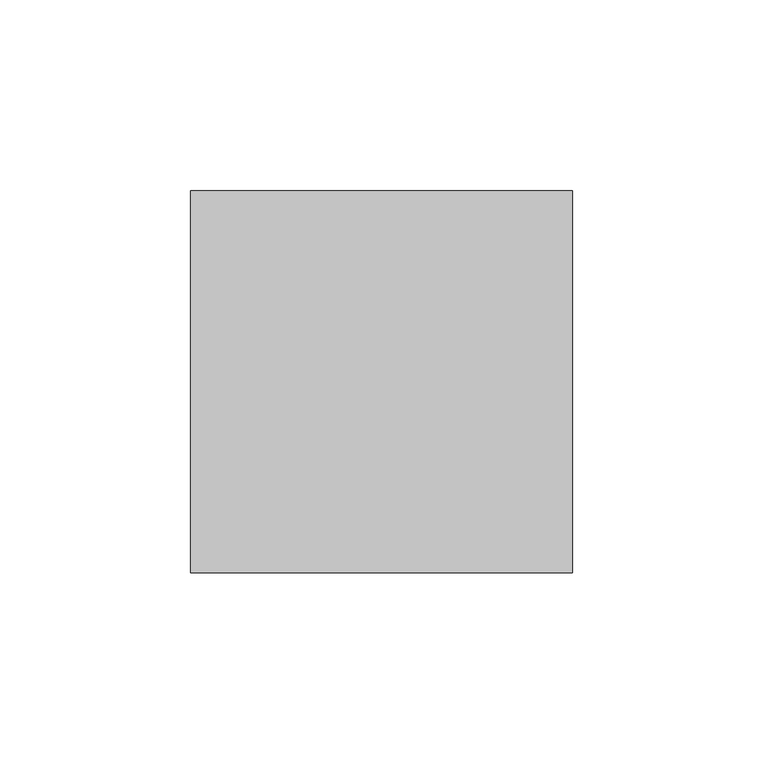
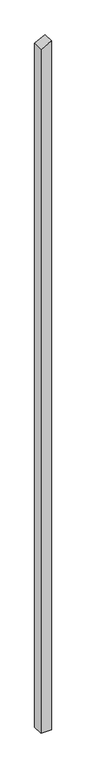
"""IFC4 building model written with IfcOpenShell, lengths in millimetres: column geometry, Holzstütze 160056 : Holzstütze 160056."""

from ifc_helpers import new_model, si_unit, frame, origin, place, context, project, spatial, polyline, outline, extrude, source, transform, mapped, element, save


def column_f815af80(model_context):
    return source(origin(), model_context, "Body", "SweptSolid", [
        extrude(outline(polyline([(-500.0, 157297.7593015), (-500.0, 157397.7593015), (6396.6643707, 157397.7593015), (6345.7118258, 157297.7593015), (-500.0, 157297.7593015)])), frame((0.0, 31941.5369795, 0.0), z_axis=(0.0, 1.0, 0.0), x_axis=(0.0, 0.0, 1.0)), (0.0, 0.0, 1.0), 100.0),
    ])


if __name__ == "__main__":
    model = new_model("IFC4")
    model_context = context("Model", 3, world=origin())
    ifc_project = project(units=[si_unit("LENGTHUNIT", "METRE", prefix="MILLI")], contexts=[model_context])
    site = spatial("IfcSite", under=ifc_project)
    building = spatial("IfcBuilding", under=site)
    placement = place(None, origin())
    column_shape = column_f815af80(model_context)
    element("IfcColumn", 1, ObjectType="Holzstütze 160056 : Holzstütze 160056", at=placement, inside=building, context=model_context, shape_type="MappedRepresentation", body=[
        mapped(column_shape, transform((0.0, 0.0, 0.0), x_axis=(1.0, 0.0, 0.0), y_axis=(0.0, 1.0, 0.0), z_axis=(0.0, 0.0, 1.0))),
    ])
    save(model, "model.ifc")

# Revit data of these elements
# Type "Holzstütze 160056 : Holzstütze 160056"
#   Abrechnungsart = "m"
#   Allright_Bauteil_ID = "0152St 0000143501"
#   Bezeichnung = "Holzstütze"
#   Codetext = "ST-HOLZ\\"
#   Gewerk = "Zimmer- und Holzbauarbeiten"
#   Material = "Holz"
#   Objektname = "Stütze"
#   NameOverride = "Holzstütze"
#   Reference = "Holzstütze"
#   Status = "NEW"
#   ThermalTransmittance = 0.0000 BTU/(h·ft²·°F)
#   Roll = 0.00°
#   Slope = 0.00°
#   2D Interaktion = yes
#   IsExternal = yes
#   LoadBearing = yes
# Element 1 (IfcColumn, "Holzstütze 160056 : Holzstütze 160056")
#   Materials on its faces: "holzschalung"
# Materials
#   "holzschalung": class "Unassigned", colour RGB 128 128 128, transparency 0
